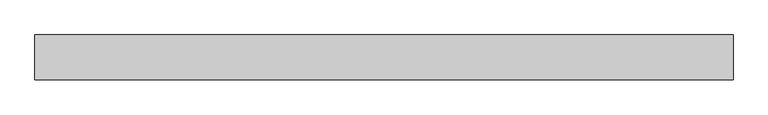
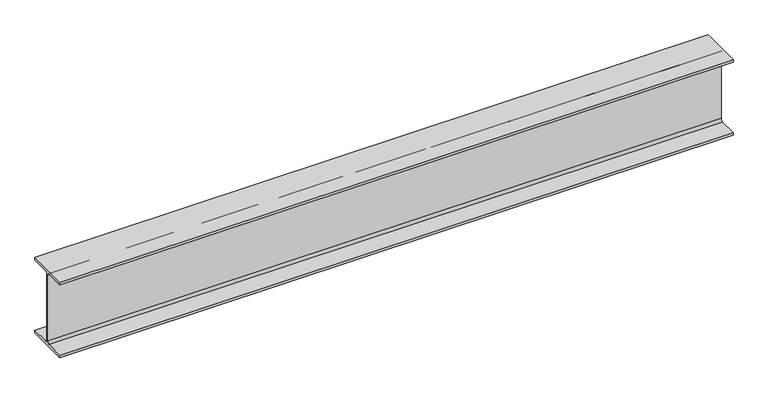
"""IFC4 building model written with IfcOpenShell, lengths in millimetres: beam geometry, Old_Steel Beam_H-KSD3502 : H_SB_ASB_H-350×175x7x11."""

from ifc_helpers import new_model, si_unit, point, frame, frame_2d, origin, place, context, project, spatial, polyline, circle_curve, trimmed, segment, composite_curve, outline, extrude, source, transform, mapped, element, save


def beam_7a789214(model_context):
    return source(origin(), model_context, "Body", "SweptSolid", [
        extrude(outline(composite_curve([segment(polyline([(82.5, -141.5), (82.5, -151.7), (-82.5, -151.7), (-82.5, -141.5), (-11.9, -141.5)]), True, "CONTINUOUS"), segment(trimmed(circle_curve(frame_2d((-11.9, -132.6)), 8.9), [point((-11.9, -141.5))], [point((-3.0, -132.6))], True, "CARTESIAN"), True, "CONTINUOUS"), segment(polyline([(-3.0, -132.6), (-3.0, 132.6)]), True, "CONTINUOUS"), segment(trimmed(circle_curve(frame_2d((-11.9, 132.6)), 8.9), [point((-3.0, 132.6))], [point((-11.9, 141.5))], True, "CARTESIAN"), True, "CONTINUOUS"), segment(polyline([(-11.9, 141.5), (-82.5, 141.5), (-82.5, 151.7), (82.5, 151.7), (82.5, 141.5), (11.9, 141.5)]), True, "CONTINUOUS"), segment(trimmed(circle_curve(frame_2d((11.9, 132.6)), 8.9), [point((11.9, 141.5))], [point((3.0, 132.6))], True, "CARTESIAN"), True, "CONTINUOUS"), segment(polyline([(3.0, 132.6), (3.0, -132.6)]), True, "CONTINUOUS"), segment(trimmed(circle_curve(frame_2d((11.9, -132.6)), 8.9), [point((3.0, -132.6))], [point((11.9, -141.5))], True, "CARTESIAN"), True, "CONTINUOUS"), segment(polyline([(11.9, -141.5), (82.5, -141.5)]), True, "CONTINUOUS")], self_intersect=False)), frame((-1295.7739051, 0.0, 0.0), z_axis=(1.0, 0.0, 0.0), x_axis=(0.0, 1.0, 0.0)), (0.0, 0.0, 1.0), 2561.6966945),
    ])


if __name__ == "__main__":
    model = new_model("IFC4")
    model_context = context("Model", 3, world=origin())
    ifc_project = project(units=[si_unit("LENGTHUNIT", "METRE", prefix="MILLI")], contexts=[model_context])
    site = spatial("IfcSite", under=ifc_project)
    building = spatial("IfcBuilding", under=site)
    placement = place(None, origin())
    beam_shape = beam_7a789214(model_context)
    element("IfcBeam", 1, ObjectType="Old_Steel Beam_H-KSD3502 : H_SB_ASB_H-350×175x7x11", at=placement, inside=building, context=model_context, shape_type="MappedRepresentation", body=[
        mapped(beam_shape, transform((0.0, 0.0, 0.0), x_axis=(1.0, 0.0, 0.0), y_axis=(0.0, 1.0, 0.0), z_axis=(0.0, 0.0, 1.0))),
    ])
    save(model, "model.ifc")

# Revit data of these elements
# Type "Old_Steel Beam_H-KSD3502 : H_SB_ASB_H-350×175x7x11"
#   Width = 17.5 cm
#   Web Thickness = 0.7 cm
#   Web Fillet = 1.4 cm
#   Warping Constant = 282290.0 cm⁶
#   Torsional Moment of Inertia = 19.4042 cm⁴
#   Torsional Modulus = 1.0 cm³
#   Section Area = 63.14 cm²
#   Plastic Modulus weak axis = 174.0 cm³
#   Plastic Modulus strong axis = 868.0 cm³
#   Perimeter = 1.36 m²/m
#   Nominal Weight = 49.60 kgf/m
#   Moment of Inertia weak axis = 984.00 cm⁴
#   Moment of Inertia strong axis = 13600.00 cm⁴
#   Height = 35.0 cm
#   Flange Thickness = 1.1 cm
#   Elastic Modulus weak axis = 112.0 cm³
#   Elastic Modulus strong axis = 775.0 cm³
#   Centroid Vertical = 17.5 cm
#   Centroid Horizontal = 8.75 cm
#   Length [instance default] = 1.5240 m
#   Structural Material [instance default] = Steel, 45-345
#   Assembly Code = ""
# Element 1 (IfcBeam, "Old_Steel Beam_H-KSD3502 : H_SB_ASB_H-350×175x7x11")
#   Structural Material = none
# Materials
#   "Steel, 45-345": class "Metal", colour RGB 189 187 185, transparency 0, Description = "Steel 345 MPa", Cost = 0
